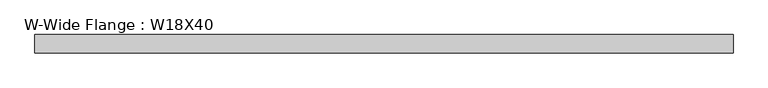
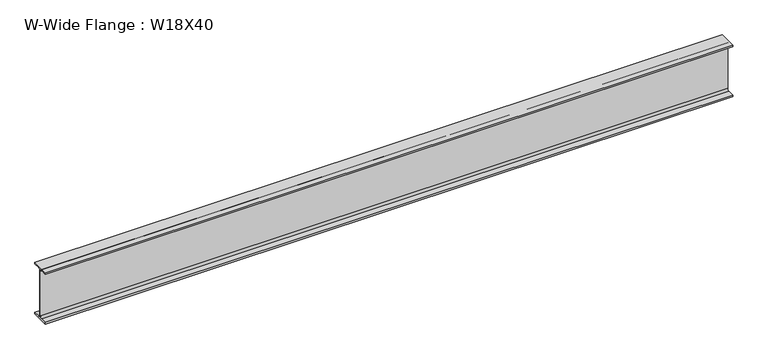
"""IFC4 building model written with IfcOpenShell, lengths in millimetres: beam geometry, W-Wide Flange : W18X40."""

from ifc_helpers import new_model, si_unit, point, frame, frame_2d, origin, place, context, project, spatial, polyline, circle_curve, trimmed, segment, composite_curve, outline, extrude, source, transform, mapped, element, save


def w_wide_flange_w18x40_03836998(model_context):
    return source(origin(), model_context, "Body", "SweptSolid", [
        extrude(outline(composite_curve([segment(polyline([(76.454, -213.995), (76.454, -227.33), (-76.454, -227.33), (-76.454, -213.995), (-20.828, -213.995)]), True, "CONTINUOUS"), segment(trimmed(circle_curve(frame_2d((-20.828, -197.1675)), 16.8275), [point((-20.828, -213.995))], [point((-4.0005, -197.1675))], True, "CARTESIAN"), True, "CONTINUOUS"), segment(polyline([(-4.0005, -197.1675), (-4.0005, 197.1675)]), True, "CONTINUOUS"), segment(trimmed(circle_curve(frame_2d((-20.828, 197.1675)), 16.8275), [point((-4.0005, 197.1675))], [point((-20.828, 213.995))], True, "CARTESIAN"), True, "CONTINUOUS"), segment(polyline([(-20.828, 213.995), (-76.454, 213.995), (-76.454, 227.33), (76.454, 227.33), (76.454, 213.995), (20.828, 213.995)]), True, "CONTINUOUS"), segment(trimmed(circle_curve(frame_2d((20.828, 197.1675)), 16.8275), [point((20.828, 213.995))], [point((4.0005, 197.1675))], True, "CARTESIAN"), True, "CONTINUOUS"), segment(polyline([(4.0005, 197.1675), (4.0005, -197.1675)]), True, "CONTINUOUS"), segment(trimmed(circle_curve(frame_2d((20.828, -197.1675)), 16.8275), [point((4.0005, -197.1675))], [point((20.828, -213.995))], True, "CARTESIAN"), True, "CONTINUOUS"), segment(polyline([(20.828, -213.995), (76.454, -213.995)]), True, "CONTINUOUS")], self_intersect=False)), frame((-2876.55, 0.0, 0.0), z_axis=(1.0, 0.0, 0.0), x_axis=(0.0, 1.0, 0.0)), (0.0, 0.0, 1.0), 5753.1),
    ])


if __name__ == "__main__":
    model = new_model("IFC4")
    model_context = context("Model", 3, world=origin())
    ifc_project = project(units=[si_unit("LENGTHUNIT", "METRE", prefix="MILLI")], contexts=[model_context])
    site = spatial("IfcSite", under=ifc_project)
    building = spatial("IfcBuilding", under=site)
    placement = place(None, origin())
    w_wide_flange_w18x40_shape = w_wide_flange_w18x40_03836998(model_context)
    element("IfcBeam", 1, ObjectType="W-Wide Flange : W18X40", at=placement, inside=building, context=model_context, shape_type="MappedRepresentation", body=[
        mapped(w_wide_flange_w18x40_shape, transform((0.0, 0.0, 0.0), x_axis=(1.0, 0.0, 0.0), y_axis=(0.0, 1.0, 0.0), z_axis=(0.0, 0.0, 1.0))),
    ])
    save(model, "model.ifc")

# Revit data of these elements
# Type "W-Wide Flange : W18X40"
#   Assembly Code = "B10"
#   W = 40
#   Length [instance default] = 5' - 0"
#   bf = 0' - 6.02"
#   d = 1' - 5.9"
#   k = 0' - 1 3/16"
#   k2 = 0' - 0.6625"
#   tf = 0' - 0.525"
#   tw = 0' - 0.315"
#   A = 0.0819444 SF
#   Structural Material [instance default] = Steel ASTM A992
# Element 1 (IfcBeam, "W-Wide Flange : W18X40")
#   Materials on its faces: "Steel ASTM A992"
# Materials
#   "Steel ASTM A992": class "Metal", colour RGB 199 199 199, transparency 0, Description = "Structural steel 50ksi", Cost = 0
